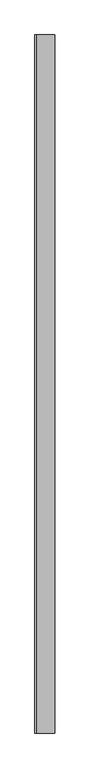
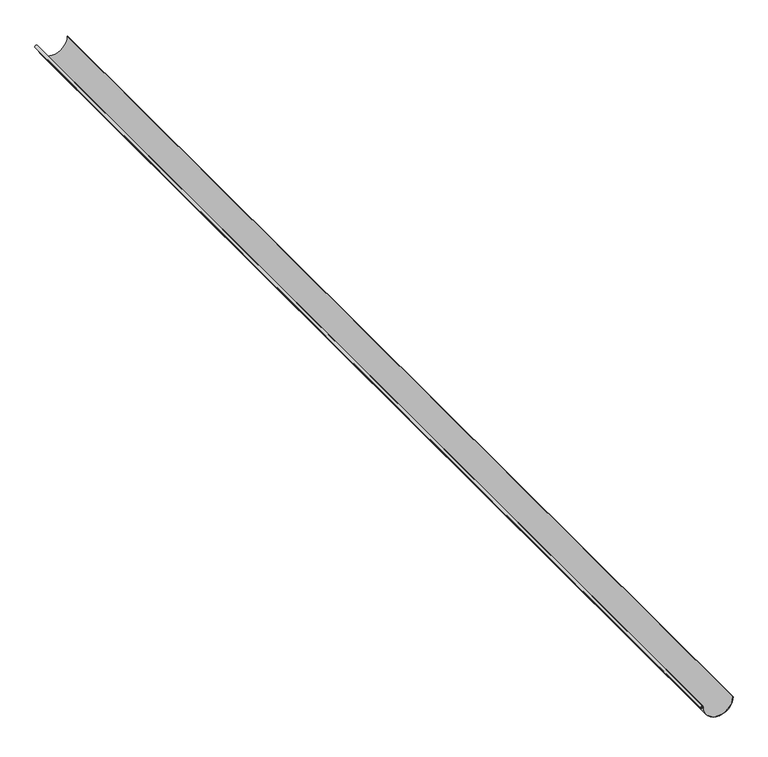
"""IFC4 building model written with IfcOpenShell, lengths in millimetres: proxy geometry, Inner panel:Inner panel:1:Inner panel:1 : Inner panel:Inner panel:300324:2:Inner panel:1:Inner panel:1 : Inner panel:Inner panel:300324:2 : Inner panel:Inner panel:1:Inner panel:1 : Inner panel:Inner panel:300324:300043:30 : Inner panel:Inner panel:1:Inner panel:1 : Inner panel:Inner panel:300324:2:Inner panel:1:Inner panel:1 : Inner panel:Inner panel:300324:2 : Inner panel:Inner panel:1:Inner panel:1 : Inner panel:Inner panel:300324:300043:308120."""

from ifc_helpers import new_model, si_unit, point, frame, frame_2d, origin, place, context, project, spatial, polyline, circle_curve, trimmed, segment, composite_curve, outline, extrude, source, transform, mapped, element, save


def generic_models_47153b61(model_context):
    return source(origin(), model_context, "Body", "SweptSolid", [
        extrude(outline(composite_curve([segment(polyline([(3815.4372291, 558129.4037733), (3815.4372291, 558127.8162733)]), True, "CONTINUOUS"), segment(trimmed(circle_curve(frame_2d((3815.4372291, 558040.5037733)), 87.3125), [point((3815.4372291, 558127.8162733))], [point((3815.4372291, 557953.1912733))], True, "CARTESIAN"), True, "CONTINUOUS"), segment(trimmed(circle_curve(frame_2d((3815.4372291, 557945.4213027)), 7.7699706), [point((3815.4372291, 557953.1912733))], [point((3809.3011565, 557950.1879636))], False, "CARTESIAN"), True, "CONTINUOUS"), segment(polyline([(3809.3011565, 557950.1879636), (3810.4348098, 557949.0543103)]), True, "CONTINUOUS"), segment(trimmed(circle_curve(frame_2d((3815.4372291, 557945.4213027)), 6.1824706), [point((3810.4348098, 557949.0543103))], [point((3815.4372291, 557951.6037733))], True, "CARTESIAN"), True, "CONTINUOUS"), segment(trimmed(circle_curve(frame_2d((3815.4372291, 558040.5037733)), 88.9), [point((3815.4372291, 557951.6037733))], [point((3815.4372291, 558129.4037733))], False, "CARTESIAN"), True, "CONTINUOUS")], self_intersect=False)), frame((0.0, -579356.0268007, 0.0), z_axis=(0.0, 1.0, 0.0), x_axis=(0.0, 0.0, 1.0)), (0.0, 0.0, 1.0), 6762.4854166),
    ])


if __name__ == "__main__":
    model = new_model("IFC4")
    model_context = context("Model", 3, world=origin())
    ifc_project = project(units=[si_unit("LENGTHUNIT", "METRE", prefix="MILLI")], contexts=[model_context])
    site = spatial("IfcSite", under=ifc_project)
    building = spatial("IfcBuilding", under=site)
    placement = place(None, origin())
    generic_models_shape = generic_models_47153b61(model_context)
    element("IfcBuildingElementProxy", 1, Name="Inner panel:Inner panel:1:Inner panel:1 : Inner panel:Inner panel:300324:2:Inner panel:1:Inner panel:1 : Inner panel:Inner panel:300324:2 : Inner panel:Inner panel:1:Inner panel:1 : Inner panel:Inner panel:300324:300043:30 : Inner panel:Inner panel:1:Inner panel:1 : Inner panel:Inner panel:300324:2:Inner panel:1:Inner panel:1 : Inner panel:Inner panel:300324:2 : Inner panel:Inner panel:1:Inner panel:1 : Inner panel:Inner panel:300324:300043:308120", ObjectType="Inner panel:Inner panel:1:Inner panel:1 : Inner panel:Inner panel:300324:2:Inner panel:1:Inner panel:1 : Inner panel:Inner panel:300324:2 : Inner panel:Inner panel:1:Inner panel:1 : Inner panel:Inner panel:300324:300043:30 : Inner panel:Inner panel:1:Inner panel:1 : Inner panel:Inner panel:300324:2:Inner panel:1:Inner panel:1 : Inner panel:Inner panel:300324:2 : Inner panel:Inner panel:1:Inner panel:1 : Inner panel:Inner panel:300324:300043:308120", at=placement, inside=building, context=model_context, shape_type="MappedRepresentation", body=[
        mapped(generic_models_shape, transform((0.0, 0.0, 0.0), x_axis=(1.0, 0.0, 0.0), y_axis=(0.0, 1.0, 0.0), z_axis=(0.0, 0.0, 1.0))),
    ])
    save(model, "model.ifc")

# Revit data of these elements
# Type "Inner panel:Inner panel:1:Inner panel:1 : Inner panel:Inner panel:300324:2:Inner panel:1:Inner panel:1 : Inner panel:Inner panel:300324:2 : Inner panel:Inner panel:1:Inner panel:1 : Inner panel:Inner panel:300324:300043:30 : Inner panel:Inner panel:1:Inner panel:1 : Inner panel:Inner panel:300324:2:Inner panel:1:Inner panel:1 : Inner panel:Inner panel:300324:2 : Inner panel:Inner panel:1:Inner panel:1 : Inner panel:Inner panel:300324:300043:308120"
#   NameOverride = "Inner panel:Inner panel:1:Inner panel:1 : Inner panel:Inner panel:300324:2:Inner panel:1:Inner panel:1 : Inner panel:Inner panel:300324:2 : Inner panel:Inner panel:1:Inner panel:1 : Inner panel:Inner panel:300324:300043:308120"
#   ObjectTypeOverride = "Inner panel:1:Inner panel:1 : Inner panel:Inner panel:300324:2 : Inner panel:Inner panel:1:Inner panel:1 : Inner panel:Inner panel:300324:300043"
#   Reference = "Inner panel"
#   Tag = "308120"
# Element 1 (IfcBuildingElementProxy, "Inner panel:Inner panel:1:Inner panel:1 : Inner panel:Inner panel:300324:2:Inner panel:1:Inner panel:1 : Inner panel:Inner panel:300324:2 : Inner panel:Inner panel:1:Inner panel:1 : Inner panel:Inner panel:300324:300043:30 : Inner panel:Inner panel:1:Inner panel:1 : Inner panel:Inner panel:300324:2:Inner panel:1:Inner panel:1 : Inner panel:Inner panel:300324:2 : Inner panel:Inner panel:1:Inner panel:1 : Inner panel:Inner panel:300324:300043:308120")
#   Materials on its faces: "HALF-ROUND GUTTERS (SLOPE TOWARD LANDSCAPING)"
# Materials
#   "HALF-ROUND GUTTERS (SLOPE TOWARD LANDSCAPING)": class "Unassigned", colour RGB 210 209 208, transparency 0, Cost = 0
